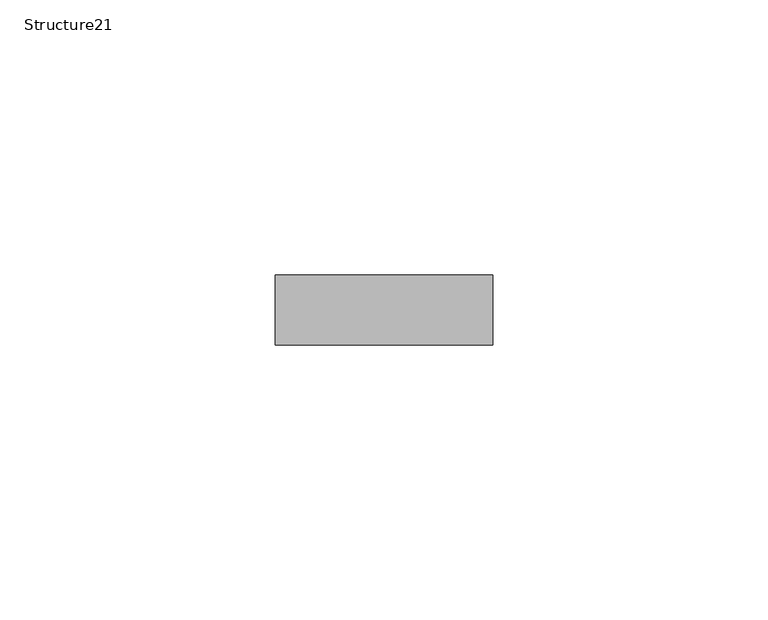
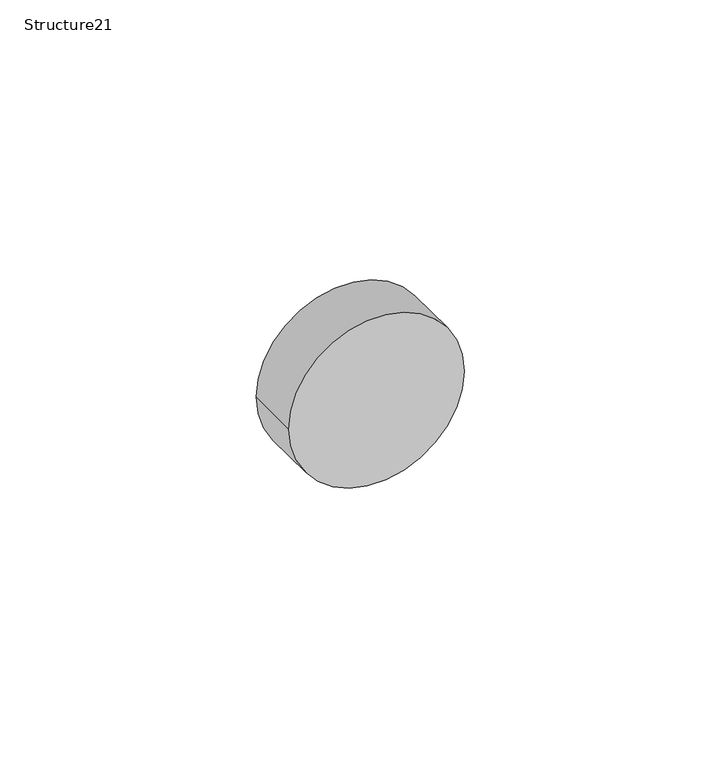
"""IFC4 building model written with IfcOpenShell, lengths in millimetres: proxy geometry, Structure21 : Structure668217149."""

from ifc_helpers import new_model, si_unit, point, frame, frame_2d, origin, place, context, project, spatial, circle_curve, trimmed, segment, composite_curve, outline, extrude, source, transform, mapped, element, save


def structure21_6640e11e(model_context):
    return source(origin(), model_context, "Body", "SweptSolid", [
        extrude(outline(composite_curve([segment(trimmed(circle_curve(frame_2d((40908.7088339, 9847.8795269)), 19.7708678), [point((40908.7088339, 9828.1086591))], [point((40908.7088339, 9867.6503947))], False, "CARTESIAN"), True, "CONTINUOUS"), segment(trimmed(circle_curve(frame_2d((40908.7088339, 9847.8795269)), 19.7708678), [point((40908.7088339, 9867.6503947))], [point((40908.7088339, 9828.1086591))], False, "CARTESIAN"), True, "CONTINUOUS")], self_intersect=False)), frame((0.0, 1964.2573723, 0.0), z_axis=(0.0, 1.0, 0.0), x_axis=(0.0, 0.0, 1.0)), (0.0, 0.0, 1.0), 12.7),
    ])


if __name__ == "__main__":
    model = new_model("IFC4")
    model_context = context("Model", 3, world=origin())
    ifc_project = project(units=[si_unit("LENGTHUNIT", "METRE", prefix="MILLI")], contexts=[model_context])
    site = spatial("IfcSite", under=ifc_project)
    building = spatial("IfcBuilding", under=site)
    placement = place(None, origin())
    structure21_shape = structure21_6640e11e(model_context)
    element("IfcBuildingElementProxy", 1, Name="Structure21 : Structure668217149", ObjectType="Structure21 : Structure668217149", at=placement, inside=building, context=model_context, shape_type="MappedRepresentation", body=[
        mapped(structure21_shape, transform((0.0, 0.0, 0.0), x_axis=(1.0, 0.0, 0.0), y_axis=(0.0, 1.0, 0.0), z_axis=(0.0, 0.0, 1.0))),
    ])
    save(model, "model.ifc")

# Revit data of these elements
# Type "Structure21 : Structure668217149"
#   NameOverride = "Structure668217149"
# Element 1 (IfcBuildingElementProxy, "Structure21 : Structure668217149")
#   Materials on its faces: "1.5\" DIA. STAINLESS STEEL RAILING"
# Materials
#   "1.5\" DIA. STAINLESS STEEL RAILING": class "Unassigned", colour RGB 128 128 128, transparency 0, Cost = 0
